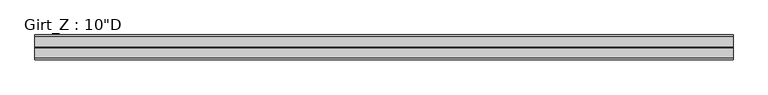
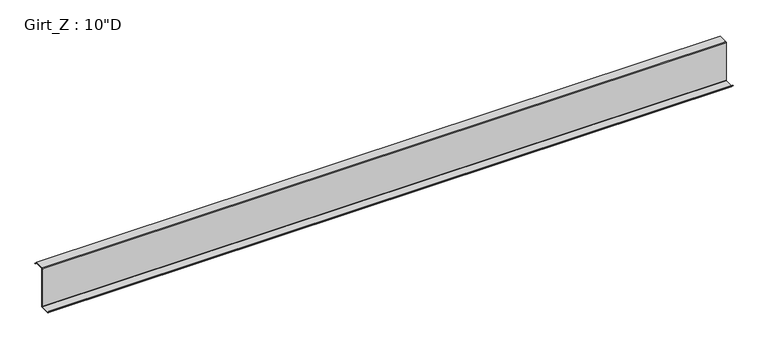
"""IFC4 building model written with IfcOpenShell, lengths in millimetres: beam geometry."""

from ifc_helpers import new_model, si_unit, point, frame, frame_2d, origin, place, context, project, spatial, polyline, circle_curve, trimmed, segment, composite_curve, outline, extrude, source, transform, mapped, element, save


def beam_1ad38590(model_context):
    return source(origin(), model_context, "Body", "SweptSolid", [
        extrude(outline(composite_curve([segment(polyline([(63.5, 127.0), (75.745104, 112.4068534), (73.6169367, 110.621109), (62.204539, 124.221875), (3.3005807, 124.221875)]), True, "CONTINUOUS"), segment(trimmed(circle_curve(frame_2d((3.3741066, 122.2381931)), 1.9850441), [point((3.3005807, 124.221875))], [point((1.3890625, 122.2381931))], True, "CARTESIAN"), True, "CONTINUOUS"), segment(polyline([(1.3890625, 122.2381931), (1.3890625, -122.2375)]), True, "CONTINUOUS"), segment(trimmed(circle_curve(frame_2d((-3.3734375, -122.2375)), 4.7625), [point((1.3890625, -122.2375))], [point((-3.3734375, -127.0))], False, "CARTESIAN"), True, "CONTINUOUS"), segment(polyline([(-3.3734375, -127.0), (-63.5, -127.0), (-75.745104, -112.4068534), (-73.6169367, -110.621109), (-62.204539, -124.221875), (-3.2694106, -124.221875)]), True, "CONTINUOUS"), segment(trimmed(circle_curve(frame_2d((-3.3748024, -122.2389339)), 1.9857399), [point((-3.2694106, -124.221875))], [point((-1.3890625, -122.2389339))], True, "CARTESIAN"), True, "CONTINUOUS"), segment(polyline([(-1.3890625, -122.2389339), (-1.3890625, 122.2375)]), True, "CONTINUOUS"), segment(trimmed(circle_curve(frame_2d((3.3734375, 122.2375)), 4.7625), [point((-1.3890625, 122.2375))], [point((3.3734375, 127.0))], False, "CARTESIAN"), True, "CONTINUOUS"), segment(polyline([(3.3734375, 127.0), (63.5, 127.0)]), True, "CONTINUOUS")], self_intersect=False)), frame((-2159.0, 0.0, 0.0), z_axis=(1.0, 0.0, 0.0), x_axis=(0.0, 1.0, 0.0)), (0.0, 0.0, 1.0), 4229.1),
    ])


if __name__ == "__main__":
    model = new_model("IFC4")
    model_context = context("Model", 3, world=origin())
    ifc_project = project(units=[si_unit("LENGTHUNIT", "METRE", prefix="MILLI")], contexts=[model_context])
    site = spatial("IfcSite", under=ifc_project)
    building = spatial("IfcBuilding", under=site)
    placement = place(None, origin())
    beam_shape = beam_1ad38590(model_context)
    element("IfcBeam", 1, ObjectType="Girt_Z : 10\"D", at=placement, inside=building, context=model_context, shape_type="MappedRepresentation", body=[
        mapped(beam_shape, transform((0.0, 0.0, 0.0), x_axis=(1.0, 0.0, 0.0), y_axis=(0.0, 1.0, 0.0), z_axis=(0.0, 0.0, 1.0))),
    ])
    save(model, "model.ifc")

# Revit data of these elements
# Type "Girt_Z : 10\"D"
#   Web_Thickness = 0' - 0 7/64"
#   Length [instance default] = 10' - 0"
#   Leg_1 = 0' - 2 1/2"
#   Height = 0' - 10"
#   Structural Material [instance default] = none
